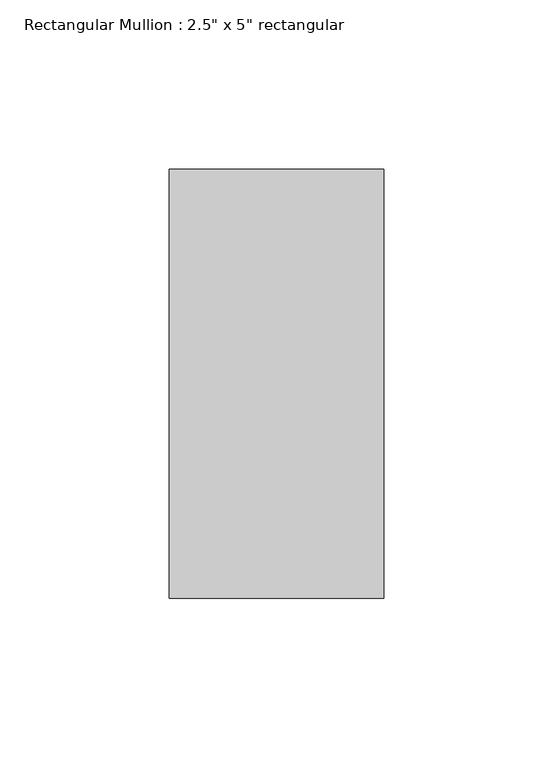
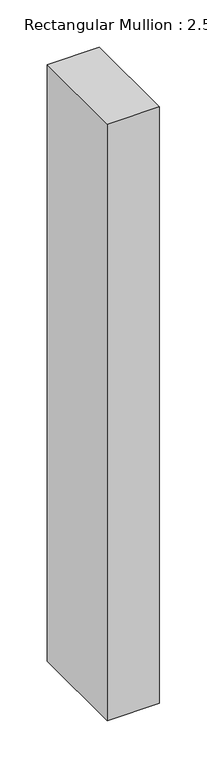
"""IFC4 building model written with IfcOpenShell, lengths in millimetres: member geometry."""

import ifcopenshell
import ifcopenshell.guid

model = None  # the IFC model being written
_history = None  # IfcOwnerHistory: only IFC2X3 demands one
_inside = {}  # id of a spatial element -> (the spatial element, [elements in it])
_under = {}  # id of a project, library or spatial element -> (it, [spatial elements below it])
_declared = {}  # id of a project -> (the project, [libraries it declares])
_typed = {}  # id of a type object -> (the type object, [elements of that type])
_made_of = {}  # id of a material, layer set ... -> (it, [elements and type objects made of it])


def new_model(schema):
    """Start an empty IFC model of exactly this schema.

    Asked for "IFC4X3", IfcOpenShell would pick the latest addendum, in which some entities
    have other attributes; the version numbers below select the first issue.
    IFC2X3 requires an IfcOwnerHistory on every rooted entity: one is made here for all.
    """
    global model, _history
    if schema == "IFC4X3":
        model = ifcopenshell.file(schema_version=(4, 3, 0, 0))
    else:
        model = ifcopenshell.file(schema=schema)
    _inside.clear()
    _under.clear()
    _declared.clear()
    _typed.clear()
    _made_of.clear()
    _history = None
    if model.schema == "IFC2X3":
        org = make("IfcOrganization", Name="unknown")
        user = make(
            "IfcPersonAndOrganization",
            ThePerson=make("IfcPerson", FamilyName="unknown"),
            TheOrganization=org,
        )
        app = make(
            "IfcApplication",
            ApplicationDeveloper=org,
            Version="unknown",
            ApplicationFullName="unknown",
            ApplicationIdentifier="unknown",
        )
        _history = make(
            "IfcOwnerHistory",
            OwningUser=user,
            OwningApplication=app,
            ChangeAction="ADDED",
            CreationDate=0,
        )
    return model


def make(cls, **values):
    """One entity of the class cls with the attributes given. An attribute that is None is left unset."""
    return model.create_entity(
        cls, **{name: value for name, value in values.items() if value is not None}
    )


def rooted(cls, **values):
    """An entity with a GlobalId (a new one), such as an element, a storey or a relation."""
    return make(cls, GlobalId=ifcopenshell.guid.new(), OwnerHistory=_history, **values)


def si_unit(unit_type, name, prefix=None):
    """IfcSIUnit, for example si_unit("LENGTHUNIT", "METRE", prefix="MILLI")."""
    return make("IfcSIUnit", UnitType=unit_type, Prefix=prefix, Name=name)


def assignment(units):
    """IfcUnitAssignment: the units of a project."""
    return None if units is None else make("IfcUnitAssignment", Units=units)


def point(xyz):
    """IfcCartesianPoint."""
    return None if xyz is None else make("IfcCartesianPoint", Coordinates=xyz)


def direction(xyz):
    """IfcDirection."""
    return None if xyz is None else make("IfcDirection", DirectionRatios=xyz)


def frame(location, z_axis=None, x_axis=None):
    """IfcAxis2Placement3D, a coordinate frame: its origin and axes. An axis left out is left unset."""
    return make(
        "IfcAxis2Placement3D",
        Location=point(location),
        Axis=direction(z_axis),
        RefDirection=direction(x_axis),
    )


def origin():
    """The frame at (0, 0, 0) with its axes left unset."""
    return frame((0.0, 0.0, 0.0))


def place(relative_to, where):
    """IfcLocalPlacement: puts the frame where relative to a parent placement (None: the world)."""
    return make(
        "IfcLocalPlacement", PlacementRelTo=relative_to, RelativePlacement=where
    )


def context(
    kind, dimensions, precision=None, world=None, true_north=None, identifier=None
):
    """IfcGeometricRepresentationContext, for example the 3D "Model" context."""
    return make(
        "IfcGeometricRepresentationContext",
        ContextIdentifier=identifier,
        ContextType=kind,
        CoordinateSpaceDimension=dimensions,
        Precision=precision,
        WorldCoordinateSystem=world,
        TrueNorth=true_north,
    )


def project(units=None, contexts=None):
    """IfcProject with its units and contexts."""
    return rooted(
        "IfcProject",
        Name="project",
        RepresentationContexts=contexts,
        UnitsInContext=assignment(units),
    )


def spatial(cls, under=None, at=None, **own):
    """A site, building, storey or space (cls), placed at a placement, below another one or the project."""
    s = rooted(cls, ObjectPlacement=at, **own)
    if under is not None:
        _under.setdefault(under.id(), (under, []))[1].append(s)
    return s


def polyline(points):
    """IfcPolyline through the points."""
    return make("IfcPolyline", Points=[point(p) for p in points])


def outline(outer, holes=None, kind="AREA"):
    """IfcArbitraryClosedProfileDef: a profile drawn as a closed curve; with holes, ...WithVoids."""
    if holes is None:
        return make("IfcArbitraryClosedProfileDef", ProfileType=kind, OuterCurve=outer)
    return make(
        "IfcArbitraryProfileDefWithVoids",
        ProfileType=kind,
        OuterCurve=outer,
        InnerCurves=holes,
    )


def extrude(swept, where, along, depth):
    """IfcExtrudedAreaSolid: the profile swept, set in the frame where, extruded along a direction by depth."""
    return make(
        "IfcExtrudedAreaSolid",
        SweptArea=swept,
        Position=where,
        ExtrudedDirection=direction(along),
        Depth=depth,
    )


def shape(context_of_items, identifier, shape_type, items):
    """IfcShapeRepresentation: the items that make up one representation, for example the "Body"."""
    return make(
        "IfcShapeRepresentation",
        ContextOfItems=context_of_items,
        RepresentationIdentifier=identifier,
        RepresentationType=shape_type,
        Items=items,
    )


def source(mapping_origin, context_of_items, identifier, shape_type, items):
    """IfcRepresentationMap: a shape defined once, which mapped items show again and again."""
    return make(
        "IfcRepresentationMap",
        MappingOrigin=mapping_origin,
        MappedRepresentation=shape(context_of_items, identifier, shape_type, items),
    )


def transform(
    local_origin,
    x_axis=None,
    y_axis=None,
    z_axis=None,
    scale=None,
    scale2=None,
    scale3=None,
    uniform=True,
):
    """IfcCartesianTransformationOperator3D, or its non-uniform kind. x_axis, y_axis, z_axis: its Axis1, 2, 3."""
    if uniform:
        return make(
            "IfcCartesianTransformationOperator3D",
            Axis1=direction(x_axis),
            Axis2=direction(y_axis),
            LocalOrigin=point(local_origin),
            Scale=scale,
            Axis3=direction(z_axis),
        )
    return make(
        "IfcCartesianTransformationOperator3DnonUniform",
        Axis1=direction(x_axis),
        Axis2=direction(y_axis),
        LocalOrigin=point(local_origin),
        Scale=scale,
        Axis3=direction(z_axis),
        Scale2=scale2,
        Scale3=scale3,
    )


def mapped(mapping_source, mapping_target):
    """IfcMappedItem: shows the shape of a source again, moved by a transform."""
    return make(
        "IfcMappedItem", MappingSource=mapping_source, MappingTarget=mapping_target
    )


def made_of(thing, what):
    """Note that an element or type object is made of a material, layer set ...; save() writes the relation."""
    if what is not None:
        _made_of.setdefault(what.id(), (what, []))[1].append(thing)
    return thing


def element(
    cls,
    number,
    at=None,
    inside=None,
    cuts=None,
    type_object=None,
    material=None,
    context=None,
    identifier="Body",
    shape_type=None,
    held_by="IfcProductDefinitionShape",
    body=None,
    shapes=None,
    **own,
):
    """One element of the class cls, such as IfcWall. Its Tag is "e" and its number.

    at: its placement. inside: the storey or other place that contains it. cuts: it is an
    opening in that element (IfcRelVoidsElement). A single representation is given by context,
    identifier, shape_type and body (its items); several are given by shapes. held_by: the class
    of the entity that holds the representations. save() writes the other relations.
    """
    e = rooted(cls, Tag="e%d" % number, ObjectPlacement=at, **own)
    if body is not None:
        shapes = [shape(context, identifier, shape_type, body)]
    if shapes is not None:
        e.Representation = make(held_by, Representations=shapes)
    if inside is not None:
        _inside.setdefault(inside.id(), (inside, []))[1].append(e)
    if cuts is not None:
        rooted(
            "IfcRelVoidsElement", RelatingBuildingElement=cuts, RelatedOpeningElement=e
        )
    if type_object is not None:
        _typed.setdefault(type_object.id(), (type_object, []))[1].append(e)
    return made_of(e, material)


def aggregate(whole, parts):
    """IfcRelAggregates: a whole, such as a stair, and the parts it consists of."""
    return rooted("IfcRelAggregates", RelatingObject=whole, RelatedObjects=parts)


def save(model, path):
    """Write the relations noted so far, then the file.

    IfcRelAggregates (storeys below a building ...), IfcRelContainedInSpatialStructure (elements
    in a storey), IfcRelDefinesByType, IfcRelAssociatesMaterial and IfcRelDeclares: one each for
    every whole, place, type object, material and project.
    """
    for whole, parts in _under.values():
        aggregate(whole, parts)
    for where, things in _inside.values():
        rooted(
            "IfcRelContainedInSpatialStructure",
            RelatedElements=things,
            RelatingStructure=where,
        )
    for kind, things in _typed.values():
        rooted("IfcRelDefinesByType", RelatedObjects=things, RelatingType=kind)
    for what, things in _made_of.values():
        rooted("IfcRelAssociatesMaterial", RelatedObjects=things, RelatingMaterial=what)
    for by, libraries in _declared.values():
        rooted("IfcRelDeclares", RelatingContext=by, RelatedDefinitions=libraries)
    model.write(path)


def member_b525e3fd(model_context):
    return source(origin(), model_context, "Body", "SweptSolid", [
        extrude(outline(polyline([(0.0, 63.5), (0.0, -63.5), (-63.5, -63.5), (-63.5, 63.5), (0.0, 63.5)])), frame((0.0, 0.0, -769.8333333), z_axis=(0.0, 0.0, 1.0), x_axis=(1.0, 0.0, 0.0)), (0.0, 0.0, 1.0), 769.8333333),
    ])


if __name__ == "__main__":
    model = new_model("IFC4")
    model_context = context("Model", 3, world=origin())
    ifc_project = project(units=[si_unit("LENGTHUNIT", "METRE", prefix="MILLI")], contexts=[model_context])
    site = spatial("IfcSite", under=ifc_project)
    building = spatial("IfcBuilding", under=site)
    placement = place(None, origin())
    member_shape = member_b525e3fd(model_context)
    element("IfcMember", 1, ObjectType="Rectangular Mullion : 2.5\" x 5\" rectangular", at=placement, inside=building, context=model_context, shape_type="MappedRepresentation", body=[
        mapped(member_shape, transform((0.0, 0.0, 0.0), x_axis=(1.0, 0.0, 0.0), y_axis=(0.0, 1.0, 0.0), z_axis=(0.0, 0.0, 1.0))),
    ])
    save(model, "model.ifc")

# Revit data of these elements
# Type "Rectangular Mullion : 2.5\" x 5\" rectangular"
#   built-in parameter 1007304 = 0.416667 (stored number, unit not read)
#   built-in parameter 1007301 = 0.104167 (stored number, unit not read)
#   built-in parameter 1007300 = 0.104167 (stored number, unit not read)
# Element 1 (IfcMember, "Rectangular Mullion : 2.5\" x 5\" rectangular")
#   Materials on its faces: "Metal - Aluminum 2"
# Materials
#   "Metal - Aluminum 2": class "Metal", colour RGB 189 187 185, transparency 0
